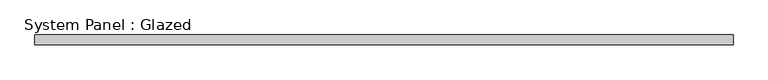
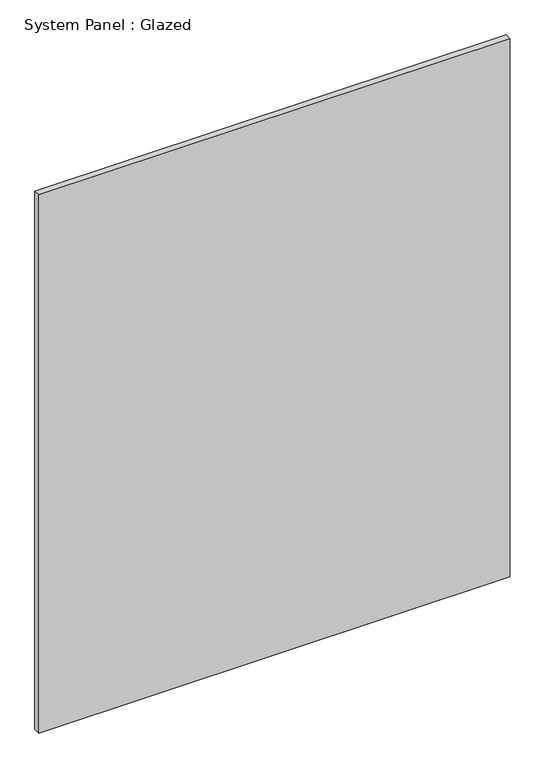
"""IFC4 building model written with IfcOpenShell, lengths in millimetres: plate geometry, System Panel : Glazed."""

from ifc_helpers import new_model, si_unit, origin, origin_with_axes, place, context, project, spatial, polyline, outline, extrude, source, transform, mapped, element, save


def system_panel_glazed_06233219(model_context):
    return source(origin(), model_context, "Body", "SweptSolid", [
        extrude(outline(polyline([(891.0, -49.5), (-891.0, -49.5), (-891.0, -24.5), (891.0, -24.5), (891.0, -49.5)])), origin_with_axes(), (0.0, 0.0, 1.0), 2150.0),
    ])


if __name__ == "__main__":
    model = new_model("IFC4")
    model_context = context("Model", 3, world=origin())
    ifc_project = project(units=[si_unit("LENGTHUNIT", "METRE", prefix="MILLI")], contexts=[model_context])
    site = spatial("IfcSite", under=ifc_project)
    building = spatial("IfcBuilding", under=site)
    placement = place(None, origin())
    system_panel_glazed_shape = system_panel_glazed_06233219(model_context)
    element("IfcPlate", 1, ObjectType="System Panel : Glazed", at=placement, inside=building, context=model_context, shape_type="MappedRepresentation", body=[
        mapped(system_panel_glazed_shape, transform((0.0, 0.0, 0.0), x_axis=(1.0, 0.0, 0.0), y_axis=(0.0, 1.0, 0.0), z_axis=(0.0, 0.0, 1.0))),
    ])
    save(model, "model.ifc")

# Revit data of these elements
# Type "System Panel : Glazed"
#   Keynote = "H11"
#   Construction Type Id = "GSP4R"
#   Analytic Construction = "1/8 in Pilkington single glazing"
#   Visual Light Transmittance = 0.9
#   Solar Heat Gain Coefficient = 0.86
#   Heat Transfer Coefficient (U) = 6.7069 W/(m²·K)
# Element 1 (IfcPlate, "System Panel : Glazed")
#   Materials on its faces: "Glass"
# Materials
#   "Glass": class "Glass", colour RGB 0 128 192, transparency 0.9, Description = "Soda Lime Glass", Cost = 0
